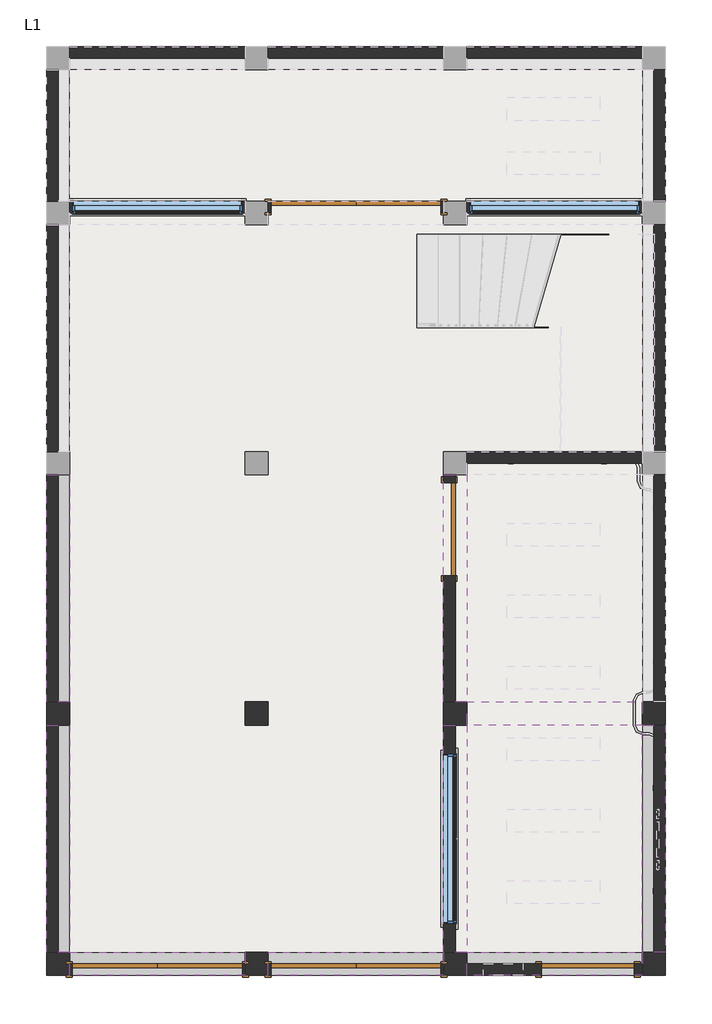
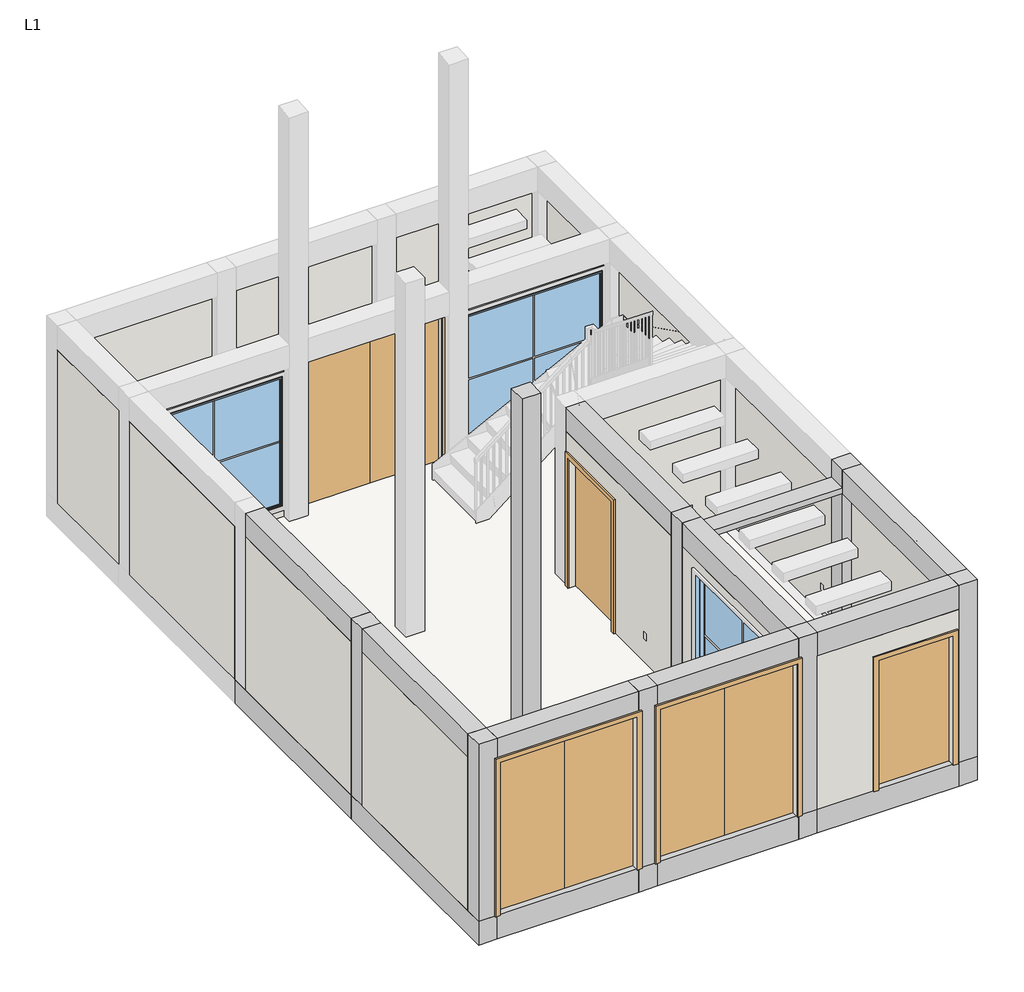
# One storey, part 1 of 3: 22 beams, 20 walls, 8 columns, 5 doors, 3 windows, 1 slab.
"""IFC4 building model written with IfcOpenShell, lengths in millimetres."""

import ifcopenshell
import ifcopenshell.guid

model = None  # the IFC model being written
_history = None  # IfcOwnerHistory: only IFC2X3 demands one
_inside = {}  # id of a spatial element -> (the spatial element, [elements in it])
_under = {}  # id of a project, library or spatial element -> (it, [spatial elements below it])
_declared = {}  # id of a project -> (the project, [libraries it declares])
_typed = {}  # id of a type object -> (the type object, [elements of that type])
_made_of = {}  # id of a material, layer set ... -> (it, [elements and type objects made of it])


def new_model(schema):
    """Start an empty IFC model of exactly this schema.

    Asked for "IFC4X3", IfcOpenShell would pick the latest addendum, in which some entities
    have other attributes; the version numbers below select the first issue.
    IFC2X3 requires an IfcOwnerHistory on every rooted entity: one is made here for all.
    """
    global model, _history
    if schema == "IFC4X3":
        model = ifcopenshell.file(schema_version=(4, 3, 0, 0))
    else:
        model = ifcopenshell.file(schema=schema)
    _inside.clear()
    _under.clear()
    _declared.clear()
    _typed.clear()
    _made_of.clear()
    _history = None
    if model.schema == "IFC2X3":
        org = make("IfcOrganization", Name="unknown")
        user = make(
            "IfcPersonAndOrganization",
            ThePerson=make("IfcPerson", FamilyName="unknown"),
            TheOrganization=org,
        )
        app = make(
            "IfcApplication",
            ApplicationDeveloper=org,
            Version="unknown",
            ApplicationFullName="unknown",
            ApplicationIdentifier="unknown",
        )
        _history = make(
            "IfcOwnerHistory",
            OwningUser=user,
            OwningApplication=app,
            ChangeAction="ADDED",
            CreationDate=0,
        )
    return model


def make(cls, **values):
    """One entity of the class cls with the attributes given. An attribute that is None is left unset."""
    return model.create_entity(
        cls, **{name: value for name, value in values.items() if value is not None}
    )


def rooted(cls, **values):
    """An entity with a GlobalId (a new one), such as an element, a storey or a relation."""
    return make(cls, GlobalId=ifcopenshell.guid.new(), OwnerHistory=_history, **values)


def si_unit(unit_type, name, prefix=None):
    """IfcSIUnit, for example si_unit("LENGTHUNIT", "METRE", prefix="MILLI")."""
    return make("IfcSIUnit", UnitType=unit_type, Prefix=prefix, Name=name)


def assignment(units):
    """IfcUnitAssignment: the units of a project."""
    return None if units is None else make("IfcUnitAssignment", Units=units)


def point(xyz):
    """IfcCartesianPoint."""
    return None if xyz is None else make("IfcCartesianPoint", Coordinates=xyz)


def direction(xyz):
    """IfcDirection."""
    return None if xyz is None else make("IfcDirection", DirectionRatios=xyz)


def frame(location, z_axis=None, x_axis=None):
    """IfcAxis2Placement3D, a coordinate frame: its origin and axes. An axis left out is left unset."""
    return make(
        "IfcAxis2Placement3D",
        Location=point(location),
        Axis=direction(z_axis),
        RefDirection=direction(x_axis),
    )


def origin():
    """The frame at (0, 0, 0) with its axes left unset."""
    return frame((0.0, 0.0, 0.0))


def origin_with_axes():
    """The frame at (0, 0, 0) with the z axis (0, 0, 1) and the x axis (1, 0, 0) written out."""
    return frame((0.0, 0.0, 0.0), z_axis=(0.0, 0.0, 1.0), x_axis=(1.0, 0.0, 0.0))


def place(relative_to, where):
    """IfcLocalPlacement: puts the frame where relative to a parent placement (None: the world)."""
    return make(
        "IfcLocalPlacement", PlacementRelTo=relative_to, RelativePlacement=where
    )


def context(
    kind, dimensions, precision=None, world=None, true_north=None, identifier=None
):
    """IfcGeometricRepresentationContext, for example the 3D "Model" context."""
    return make(
        "IfcGeometricRepresentationContext",
        ContextIdentifier=identifier,
        ContextType=kind,
        CoordinateSpaceDimension=dimensions,
        Precision=precision,
        WorldCoordinateSystem=world,
        TrueNorth=true_north,
    )


def project(units=None, contexts=None):
    """IfcProject with its units and contexts."""
    return rooted(
        "IfcProject",
        Name="project",
        RepresentationContexts=contexts,
        UnitsInContext=assignment(units),
    )


def spatial(cls, under=None, at=None, **own):
    """A site, building, storey or space (cls), placed at a placement, below another one or the project."""
    s = rooted(cls, ObjectPlacement=at, **own)
    if under is not None:
        _under.setdefault(under.id(), (under, []))[1].append(s)
    return s


def polyline(points):
    """IfcPolyline through the points."""
    return make("IfcPolyline", Points=[point(p) for p in points])


def outline(outer, holes=None, kind="AREA"):
    """IfcArbitraryClosedProfileDef: a profile drawn as a closed curve; with holes, ...WithVoids."""
    if holes is None:
        return make("IfcArbitraryClosedProfileDef", ProfileType=kind, OuterCurve=outer)
    return make(
        "IfcArbitraryProfileDefWithVoids",
        ProfileType=kind,
        OuterCurve=outer,
        InnerCurves=holes,
    )


def extrude(swept, where, along, depth):
    """IfcExtrudedAreaSolid: the profile swept, set in the frame where, extruded along a direction by depth."""
    return make(
        "IfcExtrudedAreaSolid",
        SweptArea=swept,
        Position=where,
        ExtrudedDirection=direction(along),
        Depth=depth,
    )


def faces_of(points, faces, orient=None, outer=None):
    """IfcFace entities. A face is a list of loops; a loop is a list of indices into points, from 0.

    orient and outer hold one flag for each loop. By default every Orientation is true, the
    first loop of a face is its IfcFaceOuterBound and the others are IfcFaceBound.
    """
    made = []
    for i, loops in enumerate(faces):
        bounds = []
        for j, loop in enumerate(loops):
            is_outer = j == 0 if outer is None else outer[i][j]
            bounds.append(
                make(
                    "IfcFaceOuterBound" if is_outer else "IfcFaceBound",
                    Bound=make("IfcPolyLoop", Polygon=[points[k] for k in loop]),
                    Orientation=True if orient is None else orient[i][j],
                )
            )
        made.append(make("IfcFace", Bounds=bounds))
    return made


def faceted_brep(points, faces, orient=None, outer=None, voids=None):
    """IfcFacetedBrep: a solid bounded by flat faces; with voids (closed shells), ...WithVoids."""
    shared = [point(p) for p in points]
    hull = make("IfcClosedShell", CfsFaces=faces_of(shared, faces, orient, outer))
    if voids is None:
        return make("IfcFacetedBrep", Outer=hull)
    return make(
        "IfcFacetedBrepWithVoids",
        Outer=hull,
        Voids=[
            make(cls, CfsFaces=faces_of(shared, fs, o, b)) for cls, fs, o, b in voids
        ],
    )


def shape(context_of_items, identifier, shape_type, items):
    """IfcShapeRepresentation: the items that make up one representation, for example the "Body"."""
    return make(
        "IfcShapeRepresentation",
        ContextOfItems=context_of_items,
        RepresentationIdentifier=identifier,
        RepresentationType=shape_type,
        Items=items,
    )


def source(mapping_origin, context_of_items, identifier, shape_type, items):
    """IfcRepresentationMap: a shape defined once, which mapped items show again and again."""
    return make(
        "IfcRepresentationMap",
        MappingOrigin=mapping_origin,
        MappedRepresentation=shape(context_of_items, identifier, shape_type, items),
    )


def transform(
    local_origin,
    x_axis=None,
    y_axis=None,
    z_axis=None,
    scale=None,
    scale2=None,
    scale3=None,
    uniform=True,
):
    """IfcCartesianTransformationOperator3D, or its non-uniform kind. x_axis, y_axis, z_axis: its Axis1, 2, 3."""
    if uniform:
        return make(
            "IfcCartesianTransformationOperator3D",
            Axis1=direction(x_axis),
            Axis2=direction(y_axis),
            LocalOrigin=point(local_origin),
            Scale=scale,
            Axis3=direction(z_axis),
        )
    return make(
        "IfcCartesianTransformationOperator3DnonUniform",
        Axis1=direction(x_axis),
        Axis2=direction(y_axis),
        LocalOrigin=point(local_origin),
        Scale=scale,
        Axis3=direction(z_axis),
        Scale2=scale2,
        Scale3=scale3,
    )


def mapped(mapping_source, mapping_target):
    """IfcMappedItem: shows the shape of a source again, moved by a transform."""
    return make(
        "IfcMappedItem", MappingSource=mapping_source, MappingTarget=mapping_target
    )


def made_of(thing, what):
    """Note that an element or type object is made of a material, layer set ...; save() writes the relation."""
    if what is not None:
        _made_of.setdefault(what.id(), (what, []))[1].append(thing)
    return thing


def element(
    cls,
    number,
    at=None,
    inside=None,
    cuts=None,
    type_object=None,
    material=None,
    context=None,
    identifier="Body",
    shape_type=None,
    held_by="IfcProductDefinitionShape",
    body=None,
    shapes=None,
    **own,
):
    """One element of the class cls, such as IfcWall. Its Tag is "e" and its number.

    at: its placement. inside: the storey or other place that contains it. cuts: it is an
    opening in that element (IfcRelVoidsElement). A single representation is given by context,
    identifier, shape_type and body (its items); several are given by shapes. held_by: the class
    of the entity that holds the representations. save() writes the other relations.
    """
    e = rooted(cls, Tag="e%d" % number, ObjectPlacement=at, **own)
    if body is not None:
        shapes = [shape(context, identifier, shape_type, body)]
    if shapes is not None:
        e.Representation = make(held_by, Representations=shapes)
    if inside is not None:
        _inside.setdefault(inside.id(), (inside, []))[1].append(e)
    if cuts is not None:
        rooted(
            "IfcRelVoidsElement", RelatingBuildingElement=cuts, RelatedOpeningElement=e
        )
    if type_object is not None:
        _typed.setdefault(type_object.id(), (type_object, []))[1].append(e)
    return made_of(e, material)


def aggregate(whole, parts):
    """IfcRelAggregates: a whole, such as a stair, and the parts it consists of."""
    return rooted("IfcRelAggregates", RelatingObject=whole, RelatedObjects=parts)


def save(model, path):
    """Write the relations noted so far, then the file.

    IfcRelAggregates (storeys below a building ...), IfcRelContainedInSpatialStructure (elements
    in a storey), IfcRelDefinesByType, IfcRelAssociatesMaterial and IfcRelDeclares: one each for
    every whole, place, type object, material and project.
    """
    for whole, parts in _under.values():
        aggregate(whole, parts)
    for where, things in _inside.values():
        rooted(
            "IfcRelContainedInSpatialStructure",
            RelatedElements=things,
            RelatingStructure=where,
        )
    for kind, things in _typed.values():
        rooted("IfcRelDefinesByType", RelatedObjects=things, RelatingType=kind)
    for what, things in _made_of.values():
        rooted("IfcRelAssociatesMaterial", RelatedObjects=things, RelatingMaterial=what)
    for by, libraries in _declared.values():
        rooted("IfcRelDeclares", RelatingContext=by, RelatedDefinitions=libraries)
    model.write(path)


def door_double_flush_panel_2_2_x_2_6_m_98fec84c(model_context):
    return source(origin(), model_context, "Body", "SweptSolid", [
        extrude(outline(polyline([(2600.0, -1100.0), (2600.0, 1100.0), (0.0, 1100.0), (0.0, 1176.2), (2676.2, 1176.2), (2676.2, -1176.2), (0.0, -1176.2), (0.0, -1100.0), (2600.0, -1100.0)])), frame((0.0, 75.0, 0.0), z_axis=(0.0, 1.0, 0.0), x_axis=(0.0, 0.0, 1.0)), (0.0, 0.0, 1.0), 25.4),
        extrude(outline(polyline([(2600.0, -1100.0), (2600.0, 1100.0), (0.0, 1100.0), (0.0, 1176.2), (2676.2, 1176.2), (2676.2, -1176.2), (0.0, -1176.2), (0.0, -1100.0), (2600.0, -1100.0)])), frame((0.0, -100.4, 0.0), z_axis=(0.0, 1.0, 0.0), x_axis=(0.0, 0.0, 1.0)), (0.0, 0.0, 1.0), 25.4),
        extrude(outline(polyline([(-1100.0, 75.0), (0.0, 75.0), (0.0, 24.2), (-1100.0, 24.2), (-1100.0, 75.0)])), origin_with_axes(), (0.0, 0.0, 1.0), 2600.0),
        extrude(outline(polyline([(0.0, 75.0), (1100.0, 75.0), (1100.0, 24.2), (0.0, 24.2), (0.0, 75.0)])), origin_with_axes(), (0.0, 0.0, 1.0), 2600.0),
    ])


def door_single_panel_1_2_x_2_2_m_37493633(model_context):
    return source(origin(), model_context, "Body", "SweptSolid", [
        extrude(outline(polyline([(600.0, 24.2), (-600.0, 24.2), (-600.0, 75.0), (600.0, 75.0), (600.0, 24.2)])), origin_with_axes(), (0.0, 0.0, 1.0), 2200.0),
        extrude(outline(polyline([(2276.2, 676.2), (2276.2, -676.2), (0.0, -676.2), (0.0, -600.0), (2200.0, -600.0), (2200.0, 600.0), (0.0, 600.0), (0.0, 676.2), (2276.2, 676.2)])), frame((0.0, -100.4, 0.0), z_axis=(0.0, 1.0, 0.0), x_axis=(0.0, 0.0, 1.0)), (0.0, 0.0, 1.0), 25.4),
        extrude(outline(polyline([(2276.2, -676.2), (0.0, -676.2), (0.0, -600.0), (2200.0, -600.0), (2200.0, 600.0), (0.0, 600.0), (0.0, 676.2), (2276.2, 676.2), (2276.2, -676.2)])), frame((0.0, 75.0, 0.0), z_axis=(0.0, 1.0, 0.0), x_axis=(0.0, 0.0, 1.0)), (0.0, 0.0, 1.0), 25.4),
    ])


def door_single_panel_1_2_x_2_2_m_3fbad9d7(model_context):
    return source(origin(), model_context, "Body", "SweptSolid", [
        extrude(outline(polyline([(600.0, -24.2), (600.0, -75.0), (-600.0, -75.0), (-600.0, -24.2), (600.0, -24.2)])), origin_with_axes(), (0.0, 0.0, 1.0), 2200.0),
        extrude(outline(polyline([(2276.2, 676.2), (2276.2, -676.2), (0.0, -676.2), (0.0, -600.0), (2200.0, -600.0), (2200.0, 600.0), (0.0, 600.0), (0.0, 676.2), (2276.2, 676.2)])), frame((0.0, 75.0, 0.0), z_axis=(0.0, 1.0, 0.0), x_axis=(0.0, 0.0, 1.0)), (0.0, 0.0, 1.0), 25.4),
        extrude(outline(polyline([(2276.2, -676.2), (0.0, -676.2), (0.0, -600.0), (2200.0, -600.0), (2200.0, 600.0), (0.0, 600.0), (0.0, 676.2), (2276.2, 676.2), (2276.2, -676.2)])), frame((0.0, -100.4, 0.0), z_axis=(0.0, 1.0, 0.0), x_axis=(0.0, 0.0, 1.0)), (0.0, 0.0, 1.0), 25.4),
    ])


def window_fixed_2_2_x_2_2_m_8ae7ec15(model_context):
    return source(origin(), model_context, "Body", "SolidModel", [
        faceted_brep([(1100.0, -20.25, 3114.4), (1100.0, 94.05, 3114.4), (-1100.0, 94.05, 3114.4), (-1100.0, -20.25, 3114.4), (-1100.0, 94.05, 914.4), (-1100.0, -20.25, 914.4), (1100.0, 94.05, 914.4), (1100.0, -20.25, 914.4), (1068.25, -20.25, 3082.65), (1068.25, -20.25, 946.15), (-1068.25, -20.25, 946.15), (-1068.25, -20.25, 3082.65), (-1087.3, 94.05, 3101.7), (-1087.3, 94.05, 927.1), (1087.3, 94.05, 927.1), (1087.3, 94.05, 3101.7), (1068.25, 43.25, 3082.65), (-1068.25, 43.25, 3082.65), (1087.3, 43.25, 3101.7), (-1087.3, 43.25, 3101.7), (-1068.25, 43.25, 946.15), (-1087.3, 43.25, 927.1), (1068.25, 43.25, 946.15), (1087.3, 43.25, 927.1)], [[[0, 1, 2, 3]], [[3, 2, 4, 5]], [[5, 4, 6, 7]], [[3, 5, 7, 0], [8, 9, 10, 11]], [[7, 6, 1, 0]], [[1, 6, 4, 2], [12, 13, 14, 15]], [[16, 8, 11, 17]], [[15, 18, 19, 12]], [[17, 11, 10, 20]], [[12, 19, 21, 13]], [[20, 10, 9, 22]], [[13, 21, 23, 14]], [[22, 9, 8, 16]], [[18, 23, 21, 19], [17, 20, 22, 16]], [[14, 23, 18, 15]]]),
        extrude(outline(polyline([(3114.4, -1100.0), (914.4, -1100.0), (914.4, 1100.0), (3114.4, 1100.0), (3114.4, -1100.0)]), holes=[polyline([(3101.7, 1087.3), (927.1, 1087.3), (927.1, -1087.3), (3101.7, -1087.3), (3101.7, 1087.3)])]), frame((0.0, -75.0, 0.0), z_axis=(0.0, 1.0, 0.0), x_axis=(0.0, 0.0, 1.0)), (0.0, 0.0, 1.0), 54.75),
        extrude(outline(polyline([(927.1, 1087.3), (3101.7, 1087.3), (3101.7, -1087.3), (927.1, -1087.3), (927.1, 1087.3)]), holes=[polyline([(952.5, -1061.9), (3076.3, -1061.9), (3076.3, 1061.9), (952.5, 1061.9), (952.5, -1061.9)])]), frame((0.0, 43.25, 0.0), z_axis=(0.0, 1.0, 0.0), x_axis=(0.0, 0.0, 1.0)), (0.0, 0.0, 1.0), 44.45),
        extrude(outline(polyline([(1061.9, 75.0), (1061.9, 68.65), (-1061.9, 68.65), (-1061.9, 75.0), (1061.9, 75.0)])), frame((0.0, 0.0, 952.5), z_axis=(0.0, 0.0, 1.0), x_axis=(1.0, 0.0, 0.0)), (0.0, 0.0, 1.0), 2123.8),
        extrude(outline(polyline([(-1061.9, 55.95), (-1061.9, 62.3), (1061.9, 62.3), (1061.9, 55.95), (-1061.9, 55.95)])), frame((0.0, 0.0, 952.5), z_axis=(0.0, 0.0, 1.0), x_axis=(1.0, 0.0, 0.0)), (0.0, 0.0, 1.0), 2123.8),
    ])


model = new_model("IFC4")

# Units and contexts
model_context = context("Model", 3, world=origin())
ifc_project = project(units=[si_unit("LENGTHUNIT", "METRE", prefix="MILLI")], contexts=[model_context])

# Site, building, storey
site = spatial("IfcSite", under=ifc_project)
building = spatial("IfcBuilding", under=site)
storey = spatial("IfcBuildingStorey", under=building, Name="L1", Elevation=0.0)

# Beams
placement = place(None, origin())
element("IfcBeam", 1, ObjectType="Concrete-Rectangular Beam : 30 x 40 cm", at=placement, inside=storey, context=model_context, shape_type="Brep", body=[
    faceted_brep([(-4000.0, -5500.0, 0.0), (-3700.0, -5500.0, 0.0), (-3700.0, -5200.0, 0.0), (-3700.0, -2266.6666663, 0.0), (-3700.0, -1966.6666663, 0.0), (-4000.0, -1966.6666663, 0.0), (-4000.0, -2266.6666663, 0.0), (-4000.0, -5200.0, 0.0), (-3700.0, -5500.0, -400.0), (-3700.0, -5200.0, -400.0), (-3700.0, -2266.6666663, -400.0), (-3700.0, -1966.6666663, -400.0), (-3700.0, -1966.6666663, -300.0), (-4000.0, -5500.0, -400.0), (-4000.0, -1966.6666663, -400.0)], [[[0, 1, 2, 3, 4, 5, 6, 7]], [[1, 8, 9, 10, 11, 12, 4, 3, 2]], [[8, 13, 14, 11, 10, 9]], [[13, 0, 7, 6, 5, 14]], [[1, 0, 13, 8]], [[5, 4, 12, 11, 14]]]),
])
element("IfcBeam", 2, ObjectType="Concrete-Rectangular Beam : 30 x 40 cm", at=placement, inside=storey, context=model_context, shape_type="Brep", body=[
    faceted_brep([(-3700.0, 1266.666667, 0.0), (-4000.0, 1266.666667, 0.0), (-4000.0, 966.666667, 0.0), (-4000.0, -1966.6666663, 0.0), (-3700.0, -1966.6666663, 0.0), (-3700.0, 966.666667, 0.0), (-3700.0, 1266.666667, -400.0), (-3700.0, 1266.666667, -300.0), (-3700.0, -1966.6666663, -400.0), (-3700.0, 966.666667, -400.0), (-4000.0, 1266.666667, -400.0), (-4000.0, -1966.6666663, -400.0)], [[[0, 1, 2, 3, 4, 5]], [[6, 7, 0, 5, 4, 8, 9]], [[10, 6, 9, 8, 11]], [[1, 10, 11, 3, 2]], [[1, 0, 7, 6, 10]], [[4, 3, 11, 8]]]),
])
element("IfcBeam", 3, ObjectType="Concrete-Rectangular Beam : 30 x 40 cm", at=placement, inside=storey, context=model_context, shape_type="Brep", body=[
    faceted_brep([(-1433.3333333, -5500.0, 0.0), (-1133.3333333, -5500.0, 0.0), (-1133.3333333, -5200.0, 0.0), (-1433.3333333, -5200.0, 0.0), (-1133.3333333, -5500.0, -400.0), (-1133.3333333, -5200.0, -400.0), (-1133.3333333, -2266.6666663, -400.0), (-1133.3333333, -1966.6666663, -400.0), (-1133.3333333, -1966.6666663, -300.0), (-1133.3333333, -2266.6666663, -300.0), (-1133.3333333, -5200.0, -300.0), (-1433.3333333, -5500.0, -400.0), (-1433.3333333, -5200.0, -400.0), (-1433.3333333, -2266.6666663, -400.0), (-1433.3333333, -1966.6666663, -400.0), (-1433.3333333, -5200.0, -300.0), (-1433.3333333, -2266.6666663, -300.0), (-1433.3333333, -1966.6666663, -300.0)], [[[0, 1, 2, 3]], [[1, 4, 5, 6, 7, 8, 9, 10, 2]], [[4, 11, 12, 13, 14, 7, 6, 5]], [[11, 0, 3, 15, 16, 17, 14, 13, 12]], [[1, 0, 11, 4]], [[7, 14, 17, 8]], [[15, 10, 9, 8, 17, 16]], [[10, 15, 3, 2]]]),
])
element("IfcBeam", 4, ObjectType="Concrete-Rectangular Beam : 30 x 40 cm", at=placement, inside=storey, context=model_context, shape_type="Brep", body=[
    faceted_brep([(-1133.3333333, -1966.6666663, -400.0), (-1133.3333333, 966.666667, -400.0), (-1133.3333333, 1266.666667, -400.0), (-1133.3333333, 1266.666667, -300.0), (-1133.3333333, 966.666667, -300.0), (-1133.3333333, -1966.6666663, -300.0), (-1433.3333333, 1266.666667, -400.0), (-1433.3333333, -1966.6666663, -400.0), (-1433.3333333, 966.666667, -400.0), (-1433.3333333, -1966.6666663, -300.0), (-1433.3333333, 966.666667, -300.0), (-1433.3333333, 1266.666667, -300.0)], [[[0, 1, 2, 3, 4, 5]], [[6, 2, 1, 0, 7, 8]], [[6, 8, 7, 9, 10, 11]], [[2, 6, 11, 3]], [[7, 0, 5, 9]], [[5, 4, 3, 11, 10, 9]]]),
])
element("IfcBeam", 5, ObjectType="Concrete-Rectangular Beam : 30 x 40 cm", at=placement, inside=storey, context=model_context, shape_type="Brep", body=[
    faceted_brep([(1133.33334, -5500.0, 0.0), (1433.33334, -5500.0, 0.0), (1433.33334, -5200.0, 0.0), (1133.33334, -5200.0, 0.0), (1433.33334, -5500.0, -400.0), (1433.33334, -5200.0, -400.0), (1433.33334, -2266.6666663, -400.0), (1433.33334, -1966.6666663, -400.0), (1433.33334, -1966.6666663, -300.0), (1433.33334, -2266.6666663, -300.0), (1433.33334, -5200.0, -300.0), (1133.33334, -5500.0, -400.0), (1133.33334, -5200.0, -400.0), (1133.33334, -2266.6666663, -400.0), (1133.33334, -1966.6666663, -400.0), (1133.33334, -5200.0, -300.0), (1133.33334, -2266.6666663, -300.0), (1133.33334, -1966.6666663, -300.0)], [[[0, 1, 2, 3]], [[1, 4, 5, 6, 7, 8, 9, 10, 2]], [[4, 11, 12, 13, 14, 7, 6, 5]], [[11, 0, 3, 15, 16, 17, 14, 13, 12]], [[1, 0, 11, 4]], [[7, 14, 17, 8]], [[15, 10, 9, 8, 17, 16]], [[10, 15, 3, 2]]]),
])
element("IfcBeam", 6, ObjectType="Concrete-Rectangular Beam : 30 x 40 cm", at=placement, inside=storey, context=model_context, shape_type="Brep", body=[
    faceted_brep([(1433.33334, -1966.6666663, -400.0), (1433.33334, 966.666667, -400.0), (1433.33334, 1266.666667, -400.0), (1433.33334, 1266.666667, -300.0), (1433.33334, 966.666667, -300.0), (1433.33334, -1966.6666663, -300.0), (1133.33334, 1266.666667, -400.0), (1133.33334, -1966.6666663, -400.0), (1133.33334, 966.666667, -400.0), (1133.33334, -1966.6666663, -300.0), (1133.33334, 966.666667, -300.0), (1133.33334, 1266.666667, -300.0)], [[[0, 1, 2, 3, 4, 5]], [[6, 2, 1, 0, 7, 8]], [[6, 8, 7, 9, 10, 11]], [[2, 6, 11, 3]], [[7, 0, 5, 9]], [[5, 4, 3, 11, 10, 9]]]),
])
element("IfcBeam", 7, ObjectType="Concrete-Rectangular Beam : 30 x 40 cm", at=placement, inside=storey, context=model_context, shape_type="Brep", body=[
    faceted_brep([(3700.0, -5500.0, 0.0), (4000.0, -5500.0, 0.0), (4000.0, -1966.6666663, 0.0), (3700.0, -1966.6666663, 0.0), (3700.0, -5200.0, 0.0), (4000.0, -5500.0, -400.0), (4000.0, -1966.6666663, -400.0), (3700.0, -5500.0, -400.0), (3700.0, -5200.0, -400.0), (3700.0, -2266.6666663, -400.0), (3700.0, -1966.6666663, -400.0), (3700.0, -1966.6666663, -300.0)], [[[0, 1, 2, 3, 4]], [[1, 5, 6, 2]], [[5, 7, 8, 9, 10, 6]], [[7, 0, 4, 3, 11, 10, 9, 8]], [[1, 0, 7, 5]], [[3, 2, 6, 10, 11]]]),
])
element("IfcBeam", 8, ObjectType="Concrete-Rectangular Beam : 30 x 40 cm", at=placement, inside=storey, context=model_context, shape_type="SweptSolid", body=[
    extrude(outline(polyline([(1433.33334, -2266.6666663), (1433.33334, -1966.6666663), (3700.0, -1966.6666663), (3700.0, -2266.6666663), (1433.33334, -2266.6666663)])), frame((0.0, 0.0, -400.0), z_axis=(0.0, 0.0, 1.0), x_axis=(1.0, 0.0, 0.0)), (0.0, 0.0, 1.0), 100.0),
])
element("IfcBeam", 9, ObjectType="Concrete-Rectangular Beam : 30 x 40 cm", at=placement, inside=storey, context=model_context, shape_type="SweptSolid", body=[
    extrude(outline(polyline([(-1133.3333333, -2266.6666663), (-1133.3333333, -1966.6666663), (1133.33334, -1966.6666663), (1133.33334, -2266.6666663), (-1133.3333333, -2266.6666663)])), frame((0.0, 0.0, -400.0), z_axis=(0.0, 0.0, 1.0), x_axis=(1.0, 0.0, 0.0)), (0.0, 0.0, 1.0), 100.0),
])
element("IfcBeam", 10, ObjectType="Concrete-Rectangular Beam : 30 x 40 cm", at=placement, inside=storey, context=model_context, shape_type="SweptSolid", body=[
    extrude(outline(polyline([(-3700.0, -2266.6666663), (-3700.0, -1966.6666663), (-1433.3333333, -1966.6666663), (-1433.3333333, -2266.6666663), (-3700.0, -2266.6666663)])), frame((0.0, 0.0, -400.0), z_axis=(0.0, 0.0, 1.0), x_axis=(1.0, 0.0, 0.0)), (0.0, 0.0, 1.0), 100.0),
])
element("IfcBeam", 11, ObjectType="Concrete-Rectangular Beam : 30 x 40 cm", at=placement, inside=storey, context=model_context, shape_type="Brep", body=[
    faceted_brep([(1433.33334, -5200.0, 0.0), (1433.33334, -5500.0, 0.0), (3700.0, -5500.0, 0.0), (3700.0, -5200.0, 0.0), (1433.33334, -5200.0, -400.0), (1433.33334, -5200.0, -300.0), (3700.0, -5200.0, -300.0), (3700.0, -5200.0, -400.0), (1433.33334, -5500.0, -400.0), (3700.0, -5500.0, -400.0)], [[[0, 1, 2, 3]], [[4, 5, 0, 3, 6, 7]], [[8, 4, 7, 9]], [[1, 8, 9, 2]], [[1, 0, 5, 4, 8]], [[3, 2, 9, 7, 6]]]),
])
element("IfcBeam", 12, ObjectType="Concrete-Rectangular Beam : 30 x 40 cm", at=placement, inside=storey, context=model_context, shape_type="Brep", body=[
    faceted_brep([(-1133.3333333, -5200.0, 0.0), (-1133.3333333, -5500.0, 0.0), (1133.33334, -5500.0, 0.0), (1133.33334, -5200.0, 0.0), (-1133.3333333, -5200.0, -400.0), (-1133.3333333, -5200.0, -300.0), (1133.33334, -5200.0, -300.0), (1133.33334, -5200.0, -400.0), (-1133.3333333, -5500.0, -400.0), (1133.33334, -5500.0, -400.0)], [[[0, 1, 2, 3]], [[4, 5, 0, 3, 6, 7]], [[8, 4, 7, 9]], [[1, 8, 9, 2]], [[1, 0, 5, 4, 8]], [[3, 2, 9, 7, 6]]]),
])
element("IfcBeam", 13, ObjectType="Concrete-Rectangular Beam : 30 x 40 cm", at=placement, inside=storey, context=model_context, shape_type="Brep", body=[
    faceted_brep([(-3700.0, -5200.0, 0.0), (-3700.0, -5500.0, 0.0), (-1433.3333333, -5500.0, 0.0), (-1433.3333333, -5200.0, 0.0), (-3700.0, -5200.0, -400.0), (-3700.0, -5200.0, -300.0), (-1433.3333333, -5200.0, -300.0), (-1433.3333333, -5200.0, -400.0), (-3700.0, -5500.0, -400.0), (-1433.3333333, -5500.0, -400.0)], [[[0, 1, 2, 3]], [[4, 5, 0, 3, 6, 7]], [[8, 4, 7, 9]], [[1, 8, 9, 2]], [[1, 0, 5, 4, 8]], [[3, 2, 9, 7, 6]]]),
])
element("IfcBeam", 14, ObjectType="Concrete-Rectangular Beam : 30 x 40 cm", at=placement, inside=storey, context=model_context, shape_type="SweptSolid", body=[
    extrude(outline(polyline([(-4000.0, -2266.6666663), (-3700.0, -2266.6666663), (-3700.0, -5200.0), (-4000.0, -5200.0), (-4000.0, -2266.6666663)])), frame((0.0, 0.0, 2600.0), z_axis=(0.0, 0.0, 1.0), x_axis=(1.0, 0.0, 0.0)), (0.0, 0.0, 1.0), 400.0),
])
element("IfcBeam", 15, ObjectType="Concrete-Rectangular Beam : 30 x 40 cm", at=placement, inside=storey, context=model_context, shape_type="SweptSolid", body=[
    extrude(outline(polyline([(-4000.0, 966.666667), (-3700.0, 966.666667), (-3700.0, -1966.6666663), (-4000.0, -1966.6666663), (-4000.0, 966.666667)])), frame((0.0, 0.0, 2600.0), z_axis=(0.0, 0.0, 1.0), x_axis=(1.0, 0.0, 0.0)), (0.0, 0.0, 1.0), 400.0),
])
element("IfcBeam", 16, ObjectType="Concrete-Rectangular Beam : 30 x 40 cm", at=placement, inside=storey, context=model_context, shape_type="Brep", body=[
    faceted_brep([(1433.33334, -2266.6666663, 3000.0), (1133.33334, -2266.6666663, 3000.0), (1133.33334, -5200.0, 3000.0), (1433.33334, -5200.0, 3000.0), (1433.33334, -2266.6666663, 2600.0), (1433.33334, -5200.0, 2700.0), (1433.33334, -5200.0, 2600.0), (1133.33334, -2266.6666663, 2600.0), (1133.33334, -5200.0, 2600.0)], [[[0, 1, 2, 3]], [[4, 0, 3, 5, 6]], [[7, 4, 6, 8]], [[1, 7, 8, 2]], [[1, 0, 4, 7]], [[3, 2, 8, 6, 5]]]),
])
element("IfcBeam", 17, ObjectType="Concrete-Rectangular Beam : 30 x 40 cm", at=placement, inside=storey, context=model_context, shape_type="Brep", body=[
    faceted_brep([(1433.33334, 966.666667, 3000.0), (1133.33334, 966.666667, 3000.0), (1133.33334, -1966.6666663, 3000.0), (1433.33334, -1966.6666663, 3000.0), (1433.33334, 966.666667, 2600.0), (1433.33334, 966.666667, 2700.0), (1433.33334, -1966.6666663, 2600.0), (1133.33334, 966.666667, 2600.0), (1133.33334, -1966.6666663, 2600.0)], [[[0, 1, 2, 3]], [[4, 5, 0, 3, 6]], [[7, 4, 6, 8]], [[1, 7, 8, 2]], [[1, 0, 5, 4, 7]], [[2, 8, 6, 3]]]),
])
element("IfcBeam", 18, ObjectType="Concrete-Rectangular Beam : 30 x 40 cm", at=placement, inside=storey, context=model_context, shape_type="Brep", body=[
    faceted_brep([(4000.0, -2266.6666663, 3000.0), (3700.0, -2266.6666663, 3000.0), (3700.0, -5200.0, 3000.0), (4000.0, -5200.0, 3000.0), (4000.0, -2266.6666663, 2600.0), (4000.0, -5200.0, 2600.0), (3700.0, -2266.6666663, 2600.0), (3700.0, -5200.0, 2600.0), (3700.0, -5200.0, 2700.0)], [[[0, 1, 2, 3]], [[4, 0, 3, 5]], [[6, 4, 5, 7]], [[1, 6, 7, 8, 2]], [[1, 0, 4, 6]], [[3, 2, 8, 7, 5]]]),
])
element("IfcBeam", 19, ObjectType="Concrete-Rectangular Beam : 30 x 40 cm", at=placement, inside=storey, context=model_context, shape_type="SweptSolid", body=[
    extrude(outline(polyline([(1433.33334, -2266.6666663), (1433.33334, -1966.6666663), (3699.9988976, -1966.6666663), (3699.9988976, -2266.6666663), (1433.33334, -2266.6666663)])), frame((0.0, 0.0, 2600.0), z_axis=(0.0, 0.0, 1.0), x_axis=(1.0, 0.0, 0.0)), (0.0, 0.0, 1.0), 100.0),
])
element("IfcBeam", 20, ObjectType="Concrete-Rectangular Beam : 30 x 40 cm", at=placement, inside=storey, context=model_context, shape_type="Brep", body=[
    faceted_brep([(1433.33334, -5200.0, 3000.0), (1433.33334, -5500.0, 3000.0), (3699.9988976, -5500.0, 3000.0), (3699.9988976, -5200.0, 3000.0), (1433.33334, -5200.0, 2600.0), (1433.33334, -5200.0, 2700.0), (3699.9988976, -5200.0, 2600.0), (1433.33334, -5500.0, 2600.0), (3699.9988976, -5500.0, 2600.0)], [[[0, 1, 2, 3]], [[4, 5, 0, 3, 6]], [[7, 4, 6, 8]], [[1, 7, 8, 2]], [[1, 0, 5, 4, 7]], [[3, 2, 8, 6]]]),
])
element("IfcBeam", 21, ObjectType="Concrete-Rectangular Beam : 30 x 40 cm", at=placement, inside=storey, context=model_context, shape_type="SweptSolid", body=[
    extrude(outline(polyline([(-1133.3333333, -5500.0), (-1133.3333333, -5200.0), (1133.33334, -5200.0), (1133.33334, -5500.0), (-1133.3333333, -5500.0)])), frame((0.0, 0.0, 2600.0), z_axis=(0.0, 0.0, 1.0), x_axis=(1.0, 0.0, 0.0)), (0.0, 0.0, 1.0), 400.0),
])
element("IfcBeam", 22, ObjectType="Concrete-Rectangular Beam : 30 x 40 cm", at=placement, inside=storey, context=model_context, shape_type="SweptSolid", body=[
    extrude(outline(polyline([(-3700.0, -5500.0), (-3700.0, -5200.0), (-1433.3333333, -5200.0), (-1433.3333333, -5500.0), (-3700.0, -5500.0)])), frame((0.0, 0.0, 2600.0), z_axis=(0.0, 0.0, 1.0), x_axis=(1.0, 0.0, 0.0)), (0.0, 0.0, 1.0), 400.0),
])

# Columns
element("IfcColumn", 23, ObjectType="Concrete-Square-Column : 30 x 30 cm", at=placement, inside=storey, context=model_context, shape_type="SweptSolid", body=[
    extrude(outline(polyline([(-4000.0, -2266.6666663), (-4000.0, -1966.6666663), (-3700.0, -1966.6666663), (-3700.0, -2266.6666663), (-4000.0, -2266.6666663)])), origin_with_axes(), (0.0, 0.0, 1.0), 3000.0),
])
element("IfcColumn", 24, ObjectType="Concrete-Square-Column : 30 x 30 cm", at=placement, inside=storey, context=model_context, shape_type="SweptSolid", body=[
    extrude(outline(polyline([(-1433.3333333, -2266.6666663), (-1433.3333333, -1966.6666663), (-1133.3333333, -1966.6666663), (-1133.3333333, -2266.6666663), (-1433.3333333, -2266.6666663)])), origin_with_axes(), (0.0, 0.0, 1.0), 6000.0),
])
element("IfcColumn", 25, ObjectType="Concrete-Square-Column : 30 x 30 cm", at=placement, inside=storey, context=model_context, shape_type="SweptSolid", body=[
    extrude(outline(polyline([(1133.33334, -2266.6666663), (1133.33334, -1966.6666663), (1433.33334, -1966.6666663), (1433.33334, -2266.6666663), (1133.33334, -2266.6666663)])), origin_with_axes(), (0.0, 0.0, 1.0), 3000.0),
])
element("IfcColumn", 26, ObjectType="Concrete-Square-Column : 30 x 30 cm", at=placement, inside=storey, context=model_context, shape_type="SweptSolid", body=[
    extrude(outline(polyline([(3699.9988976, -2266.6666663), (3699.9988976, -1966.6666663), (3999.9988976, -1966.6666663), (3999.9988976, -2266.6666663), (3699.9988976, -2266.6666663)])), origin_with_axes(), (0.0, 0.0, 1.0), 3000.0),
])
element("IfcColumn", 27, ObjectType="Concrete-Square-Column : 30 x 30 cm", at=placement, inside=storey, context=model_context, shape_type="SweptSolid", body=[
    extrude(outline(polyline([(-4000.0, -5500.0), (-4000.0, -5200.0), (-3700.0, -5200.0), (-3700.0, -5500.0), (-4000.0, -5500.0)])), origin_with_axes(), (0.0, 0.0, 1.0), 3000.0),
])
element("IfcColumn", 28, ObjectType="Concrete-Square-Column : 30 x 30 cm", at=placement, inside=storey, context=model_context, shape_type="SweptSolid", body=[
    extrude(outline(polyline([(-1433.3333333, -5500.0), (-1433.3333333, -5200.0), (-1133.3333333, -5200.0), (-1133.3333333, -5500.0), (-1433.3333333, -5500.0)])), origin_with_axes(), (0.0, 0.0, 1.0), 3000.0),
])
element("IfcColumn", 29, ObjectType="Concrete-Square-Column : 30 x 30 cm", at=placement, inside=storey, context=model_context, shape_type="SweptSolid", body=[
    extrude(outline(polyline([(1133.33334, -5500.0), (1133.33334, -5200.0), (1433.33334, -5200.0), (1433.33334, -5500.0), (1133.33334, -5500.0)])), origin_with_axes(), (0.0, 0.0, 1.0), 3000.0),
])
element("IfcColumn", 30, ObjectType="Concrete-Square-Column : 30 x 30 cm", at=placement, inside=storey, context=model_context, shape_type="SweptSolid", body=[
    extrude(outline(polyline([(3699.9988976, -5500.0), (3699.9988976, -5200.0), (3999.9988976, -5200.0), (3999.9988976, -5500.0), (3699.9988976, -5500.0)])), origin_with_axes(), (0.0, 0.0, 1.0), 3000.0),
])

# Doors
door_double_flush_panel_2_2_x_2_6_m_shape = door_double_flush_panel_2_2_x_2_6_m_98fec84c(model_context)
element("IfcDoor", 31, ObjectType="Door-Double-Flush_Panel : 2.2 x 2.6 m", at=placement, inside=storey, context=model_context, shape_type="MappedRepresentation", body=[
    mapped(door_double_flush_panel_2_2_x_2_6_m_shape, transform((-2566.6666667, -5425.0, 0.0), x_axis=(1.0, 0.0, 0.0), y_axis=(0.0, 1.0, 0.0), z_axis=(0.0, 0.0, 1.0))),
])
element("IfcDoor", 32, ObjectType="Door-Double-Flush_Panel : 2.2 x 2.6 m", at=placement, inside=storey, context=model_context, shape_type="MappedRepresentation", body=[
    mapped(door_double_flush_panel_2_2_x_2_6_m_shape, transform((3.3e-06, -5425.0, 0.0), x_axis=(1.0, 0.0, 0.0), y_axis=(0.0, 1.0, 0.0), z_axis=(0.0, 0.0, 1.0))),
])
element("IfcDoor", 33, ObjectType="Door-Double-Flush_Panel : 2.2 x 2.6 m", at=placement, inside=storey, context=model_context, shape_type="MappedRepresentation", body=[
    mapped(door_double_flush_panel_2_2_x_2_6_m_shape, transform((3.3e-06, 4425.0, 0.0), x_axis=(1.0, 0.0, 0.0), y_axis=(0.0, 1.0, 0.0), z_axis=(0.0, 0.0, 1.0))),
])
door_single_panel_1_2_x_2_2_m_shape = door_single_panel_1_2_x_2_2_m_37493633(model_context)
element("IfcDoor", 34, ObjectType="Door-Single-Panel : 1.2 x 2.2 m", at=placement, inside=storey, context=model_context, shape_type="MappedRepresentation", body=[
    mapped(door_single_panel_1_2_x_2_2_m_shape, transform((3000.0, -5425.0, 0.0), x_axis=(1.0, 0.0, 0.0), y_axis=(0.0, 1.0, 0.0), z_axis=(0.0, 0.0, 1.0))),
])
door_single_panel_1_2_x_2_2_m_2_shape = door_single_panel_1_2_x_2_2_m_3fbad9d7(model_context)
element("IfcDoor", 35, ObjectType="Door-Single-Panel : 1.2 x 2.2 m", at=placement, inside=storey, context=model_context, shape_type="MappedRepresentation", body=[
    mapped(door_single_panel_1_2_x_2_2_m_2_shape, transform((1208.33334, 266.666667, 0.0), x_axis=(0.0, 1.0, 0.0), y_axis=(-1.0, 0.0, 0.0), z_axis=(0.0, 0.0, 1.0))),
])

# Slab
element("IfcSlab", 36, ObjectType="Genérico 300 mm", at=placement, inside=storey, context=model_context, shape_type="Brep", body=[
    faceted_brep([(3700.0, 6200.0, -300.0), (3700.0, 4500.0, -300.0), (3700.0, 4200.0, -300.0), (3700.0, 1266.666667, -300.0), (3700.0, 966.666667, -300.0), (3700.0, -1966.6666663, -300.0), (3700.0, -2266.6666663, -300.0), (3700.0, -5200.0, -300.0), (1433.33334, -5200.0, -300.0), (1133.33334, -5200.0, -300.0), (-1133.3333333, -5200.0, -300.0), (-1433.3333333, -5200.0, -300.0), (-3700.0, -5200.0, -300.0), (-3700.0, -2266.6666663, -300.0), (-3700.0, -1966.6666663, -300.0), (-3700.0, 966.666667, -300.0), (-3700.0, 1266.666667, -300.0), (-3700.0, 4200.0, -300.0), (-3700.0, 4500.0, -300.0), (-3700.0, 6200.0, -300.0), (-1433.3333333, 6200.0, -300.0), (-1133.3333333, 6200.0, -300.0), (1133.33334, 6200.0, -300.0), (1433.33334, 6200.0, -300.0), (3700.0, 6200.0, 0.0), (1433.33334, 6200.0, 0.0), (1133.33334, 6200.0, 0.0), (-1133.3333333, 6200.0, 0.0), (-1433.3333333, 6200.0, 0.0), (-3700.0, 6200.0, 0.0), (-3700.0, 4500.0, 0.0), (-3700.0, 1266.666667, 0.0), (-3700.0, -1966.6666663, 0.0), (-3700.0, -5200.0, 0.0), (-1433.3333333, -5200.0, 0.0), (-1133.3333333, -5200.0, 0.0), (1133.33334, -5200.0, 0.0), (1433.33334, -5200.0, 0.0), (3700.0, -5200.0, 0.0), (3700.0, -1966.6666663, 0.0), (3700.0, 1266.666667, 0.0), (3700.0, 4500.0, 0.0)], [[[0, 1, 2, 3, 4, 5, 6, 7, 8, 9, 10, 11, 12, 13, 14, 15, 16, 17, 18, 19, 20, 21, 22, 23]], [[24, 25, 26, 27, 28, 29, 30, 31, 32, 33, 34, 35, 36, 37, 38, 39, 40, 41]], [[7, 6, 5, 4, 3, 2, 1, 0, 24, 41, 40, 39, 38]], [[12, 11, 10, 9, 8, 7, 38, 37, 36, 35, 34, 33]], [[19, 18, 17, 16, 15, 14, 13, 12, 33, 32, 31, 30, 29]], [[0, 23, 22, 21, 20, 19, 29, 28, 27, 26, 25, 24]]]),
])

# Walls
element("IfcWall", 37, ObjectType="Genérico - 150 mm", at=placement, inside=storey, context=model_context, shape_type="SweptSolid", body=[
    extrude(outline(polyline([(0.0, 3700.0), (2600.0, 3700.0), (2600.0, 1433.33334), (0.0, 1433.33334), (0.0, 2400.0), (2200.0, 2400.0), (2200.0, 3600.0), (0.0, 3600.0), (0.0, 3700.0)])), frame((0.0, -5500.0, 0.0), z_axis=(0.0, 1.0, 0.0), x_axis=(0.0, 0.0, 1.0)), (0.0, 0.0, 1.0), 150.0),
])
element("IfcWall", 38, ObjectType="Genérico - 150 mm", at=placement, inside=storey, context=model_context, shape_type="SweptSolid", body=[
    extrude(outline(polyline([(4000.0, -2266.6666663), (4000.0, -5200.0), (3850.0, -5200.0), (3850.0, -2266.6666663), (4000.0, -2266.6666663)])), origin_with_axes(), (0.0, 0.0, 1.0), 2600.0),
])
element("IfcWall", 39, ObjectType="Genérico - 150 mm", at=placement, inside=storey, context=model_context, shape_type="SweptSolid", body=[
    extrude(outline(polyline([(4000.0, 966.666667), (4000.0, -1966.6666663), (3850.0, -1966.6666663), (3850.0, 966.666667), (4000.0, 966.666667)])), origin_with_axes(), (0.0, 0.0, 1.0), 2600.0),
])
element("IfcWall", 40, ObjectType="Genérico - 150 mm", at=placement, inside=storey, context=model_context, shape_type="SweptSolid", body=[
    extrude(outline(polyline([(4000.0, 4200.0), (4000.0, 1266.666667), (3850.0, 1266.666667), (3850.0, 4200.0), (4000.0, 4200.0)])), origin_with_axes(), (0.0, 0.0, 1.0), 2600.0),
])
element("IfcWall", 41, ObjectType="Genérico - 150 mm", at=placement, inside=storey, context=model_context, shape_type="SweptSolid", body=[
    extrude(outline(polyline([(4000.0, 6200.0), (4000.0, 4500.0), (3850.0, 4500.0), (3850.0, 6200.0), (4000.0, 6200.0)])), origin_with_axes(), (0.0, 0.0, 1.0), 2600.0),
])
element("IfcWall", 42, ObjectType="Genérico - 150 mm", at=placement, inside=storey, context=model_context, shape_type="SweptSolid", body=[
    extrude(outline(polyline([(1433.33334, 6500.0), (3700.0, 6500.0), (3700.0, 6350.0), (1433.33334, 6350.0), (1433.33334, 6500.0)])), origin_with_axes(), (0.0, 0.0, 1.0), 2600.0),
])
element("IfcWall", 43, ObjectType="Genérico - 150 mm", at=placement, inside=storey, context=model_context, shape_type="SweptSolid", body=[
    extrude(outline(polyline([(-1433.3333333, -5350.0), (-1433.3333333, -5500.0), (-1466.6666667, -5500.0), (-1466.6666667, -5350.0), (-1433.3333333, -5350.0)])), origin_with_axes(), (0.0, 0.0, 1.0), 2600.0),
    extrude(outline(polyline([(-3700.0, -5500.0), (-3700.0, -5350.0), (-3666.6666667, -5350.0), (-3666.6666667, -5500.0), (-3700.0, -5500.0)])), origin_with_axes(), (0.0, 0.0, 1.0), 2600.0),
])
element("IfcWall", 44, ObjectType="Genérico - 150 mm", at=placement, inside=storey, context=model_context, shape_type="SweptSolid", body=[
    extrude(outline(polyline([(1133.33334, -5350.0), (1133.33334, -5500.0), (1100.0000033, -5500.0), (1100.0000033, -5350.0), (1133.33334, -5350.0)])), origin_with_axes(), (0.0, 0.0, 1.0), 2600.0),
    extrude(outline(polyline([(-1133.3333333, -5500.0), (-1133.3333333, -5350.0), (-1099.9999967, -5350.0), (-1099.9999967, -5500.0), (-1133.3333333, -5500.0)])), origin_with_axes(), (0.0, 0.0, 1.0), 2600.0),
])
element("IfcWall", 45, ObjectType="Genérico - 150 mm", at=placement, inside=storey, context=model_context, shape_type="SweptSolid", body=[
    extrude(outline(polyline([(-3850.0, -2266.6666663), (-3850.0, -5200.0), (-4000.0, -5200.0), (-4000.0, -2266.6666663), (-3850.0, -2266.6666663)])), origin_with_axes(), (0.0, 0.0, 1.0), 2600.0),
])
element("IfcWall", 46, ObjectType="Genérico - 150 mm", at=placement, inside=storey, context=model_context, shape_type="SweptSolid", body=[
    extrude(outline(polyline([(-3850.0, 966.666667), (-3850.0, -1966.6666663), (-4000.0, -1966.6666663), (-4000.0, 966.666667), (-3850.0, 966.666667)])), origin_with_axes(), (0.0, 0.0, 1.0), 2600.0),
])
element("IfcWall", 47, ObjectType="Genérico - 150 mm", at=placement, inside=storey, context=model_context, shape_type="SweptSolid", body=[
    extrude(outline(polyline([(-3850.0, 4200.0), (-3850.0, 1266.666667), (-4000.0, 1266.666667), (-4000.0, 4200.0), (-3850.0, 4200.0)])), origin_with_axes(), (0.0, 0.0, 1.0), 2600.0),
])
element("IfcWall", 48, ObjectType="Genérico - 150 mm", at=placement, inside=storey, context=model_context, shape_type="SweptSolid", body=[
    extrude(outline(polyline([(-3850.0, 6200.0), (-3850.0, 4500.0), (-4000.0, 4500.0), (-4000.0, 6200.0), (-3850.0, 6200.0)])), origin_with_axes(), (0.0, 0.0, 1.0), 2600.0),
])
element("IfcWall", 49, ObjectType="Genérico - 150 mm", at=placement, inside=storey, context=model_context, shape_type="SweptSolid", body=[
    extrude(outline(polyline([(-1433.3333333, 6350.0), (-3700.0, 6350.0), (-3700.0, 6500.0), (-1433.3333333, 6500.0), (-1433.3333333, 6350.0)])), origin_with_axes(), (0.0, 0.0, 1.0), 2600.0),
])
element("IfcWall", 50, ObjectType="Genérico - 150 mm", at=placement, inside=storey, context=model_context, shape_type="SweptSolid", body=[
    extrude(outline(polyline([(1133.33334, 6350.0), (-1133.3333333, 6350.0), (-1133.3333333, 6500.0), (1133.33334, 6500.0), (1133.33334, 6350.0)])), origin_with_axes(), (0.0, 0.0, 1.0), 2600.0),
])
element("IfcWall", 51, ObjectType="Genérico - 150 mm", at=placement, inside=storey, context=model_context, shape_type="SweptSolid", body=[
    extrude(outline(polyline([(0.0, -3700.0), (0.0, -1433.3333333), (2600.0, -1433.3333333), (2600.0, -3700.0), (0.0, -3700.0)]), holes=[polyline([(200.0, -3666.6666667), (2400.0, -3666.6666667), (2400.0, -1466.6666667), (200.0, -1466.6666667), (200.0, -3666.6666667)])]), frame((0.0, 4350.0, 0.0), z_axis=(0.0, 1.0, 0.0), x_axis=(0.0, 0.0, 1.0)), (0.0, 0.0, 1.0), 150.0),
])
element("IfcWall", 52, ObjectType="Genérico - 150 mm", at=placement, inside=storey, context=model_context, shape_type="SweptSolid", body=[
    extrude(outline(polyline([(1133.33334, 4500.0), (1133.33334, 4350.0), (1100.0000033, 4350.0), (1100.0000033, 4500.0), (1133.33334, 4500.0)])), origin_with_axes(), (0.0, 0.0, 1.0), 2600.0),
    extrude(outline(polyline([(-1133.3333333, 4350.0), (-1133.3333333, 4500.0), (-1099.9999967, 4500.0), (-1099.9999967, 4350.0), (-1133.3333333, 4350.0)])), origin_with_axes(), (0.0, 0.0, 1.0), 2600.0),
])
element("IfcWall", 53, ObjectType="Genérico - 150 mm", at=placement, inside=storey, context=model_context, shape_type="SweptSolid", body=[
    extrude(outline(polyline([(0.0, 1433.33334), (0.0, 3700.0), (2600.0, 3700.0), (2600.0, 1433.33334), (0.0, 1433.33334)]), holes=[polyline([(200.0, 1466.66667), (2400.0, 1466.66667), (2400.0, 3666.66667), (200.0, 3666.66667), (200.0, 1466.66667)])]), frame((0.0, 4350.0, 0.0), z_axis=(0.0, 1.0, 0.0), x_axis=(0.0, 0.0, 1.0)), (0.0, 0.0, 1.0), 150.0),
])
element("IfcWall", 54, ObjectType="Genérico - 150 mm", at=placement, inside=storey, context=model_context, shape_type="SweptSolid", body=[
    extrude(outline(polyline([(3700.0, 1116.666667), (1433.33334, 1116.666667), (1433.33334, 1266.666667), (3700.0, 1266.666667), (3700.0, 1116.666667)])), origin_with_axes(), (0.0, 0.0, 1.0), 2600.0),
])
element("IfcWall", 55, ObjectType="Genérico - 150 mm", at=placement, inside=storey, context=model_context, shape_type="SweptSolid", body=[
    extrude(outline(polyline([(966.666667, 0.0), (866.666667, 0.0), (866.666667, 2200.0), (-333.333333, 2200.0), (-333.333333, 0.0), (-1966.6666663, 0.0), (-1966.6666663, 2600.0), (966.666667, 2600.0), (966.666667, 0.0)])), frame((1133.33334, 0.0, 0.0), z_axis=(1.0, 0.0, 0.0), x_axis=(0.0, 1.0, 0.0)), (0.0, 0.0, 1.0), 150.0),
])
element("IfcWall", 56, ObjectType="Genérico - 150 mm", at=placement, inside=storey, context=model_context, shape_type="SweptSolid", body=[
    extrude(outline(polyline([(-2266.6666663, 0.0), (-5200.0, 0.0), (-5200.0, 2600.0), (-2266.6666663, 2600.0), (-2266.6666663, 0.0)]), holes=[polyline([(-4833.3333332, 2400.0), (-4833.3333332, 200.0), (-2633.3333332, 200.0), (-2633.3333332, 2400.0), (-4833.3333332, 2400.0)])]), frame((1133.33334, 0.0, 0.0), z_axis=(1.0, 0.0, 0.0), x_axis=(0.0, 1.0, 0.0)), (0.0, 0.0, 1.0), 150.0),
])

# Windows
window_fixed_2_2_x_2_2_m_shape = window_fixed_2_2_x_2_2_m_8ae7ec15(model_context)
element("IfcWindow", 57, ObjectType="Window-Fixed : 2.2 x 2.2 m", at=placement, inside=storey, context=model_context, shape_type="MappedRepresentation", body=[
    mapped(window_fixed_2_2_x_2_2_m_shape, transform((1208.33334, -3733.3333332, -714.4), x_axis=(0.0, -1.0, 0.0), y_axis=(1.0, 0.0, 0.0), z_axis=(0.0, 0.0, 1.0))),
])
element("IfcWindow", 58, ObjectType="Window-Fixed : 2.2 x 2.2 m", at=placement, inside=storey, context=model_context, shape_type="MappedRepresentation", body=[
    mapped(window_fixed_2_2_x_2_2_m_shape, transform((-2566.6666667, 4425.0, -714.4), x_axis=(-1.0, 0.0, 0.0), y_axis=(0.0, -1.0, 0.0), z_axis=(0.0, 0.0, 1.0))),
])
element("IfcWindow", 59, ObjectType="Window-Fixed : 2.2 x 2.2 m", at=placement, inside=storey, context=model_context, shape_type="MappedRepresentation", body=[
    mapped(window_fixed_2_2_x_2_2_m_shape, transform((2566.66667, 4425.0, -714.4), x_axis=(-1.0, 0.0, 0.0), y_axis=(0.0, -1.0, 0.0), z_axis=(0.0, 0.0, 1.0))),
])

save(model, "model.ifc")

# Revit data of these elements
# Project information
#   Organization Name = "Nombre de organización"
#   Organization Description = "Descripción de organización"
#   Building Name = "Nombre del edificio"
#   Project Issue Date = "Fecha de emisión"
#   Project Status = "Estado de proyecto"
#   Client Name = "Nombre de cliente"
#   Project Address = "Introduzca la dirección aquí\nLínea de dirección 2"
#   Project Name = "Nombre de proyecto"
#   Project Number = "Número de proyecto"
# Grids (mm)
#   "A": line (-3850, 7871.57) -> (-3850, -5500)
#   "1": line (-5800.121, 6350) -> (5655.078, 6350)
#   "2": line (-5800.121, 4350) -> (5655.078, 4350)
#   "3": line (-5800.121, 1116.667) -> (5655.078, 1116.667)
#   "4": line (-5800.121, -2116.667) -> (5655.078, -2116.667)
#   "B": line (-1283.333, 7871.57) -> (-1283.333, -5500)
#   "C": line (1283.333, 7871.57) -> (1283.333, -5500)
#   "D": line (3849.999, 7871.57) -> (3849.999, -5500)
#   "5": line (-5800.121, -5350) -> (5655.078, -5350)
# Type "Concrete-Rectangular Beam : 30 x 40 cm"
#   Length [instance default] = 1.524 m
#   b = 0.3 m
#   h = 0.4 m
#   Structural Material [instance default] = Concrete, Cast-in-Place gray
#   Assembly Code = ""
# Type "Concrete-Square-Column : 30 x 30 cm"
#   b = 0.3 m
#   Structural Material [instance default] = Concrete, Cast-in-Place gray
# Type "Door-Double-Flush_Panel : 2.2 x 2.6 m"
#   Type Mark = "49"
#   Construction Type Id = "DOOR"
#   Analytic Construction = "Wooden"
#   Thickness = 0.0508 m
#   Thermal Resistance (R) = 0.455703 (m²·K)/W
#   Swing Angle [instance default] = 90.00°
#   Panel Width = 1.1 m
#   Heat Transfer Coefficient (U) = 2.19465 W/(m²·K)
#   Height = 2.6 m
#   Trim Projection Ext = 0.0254 m
#   Trim Projection Int = 0.0254 m
#   Trim Width = 0.0762 m
#   Width = 2.2 m
#   Define Thermal Properties by = 1
#   Panel Material = Wood - Birch - Solid Stained Light Low Gloss
#   Trim Material = Paint - Sienna
#   Visual Light Transmittance = 0
#   Solar Heat Gain Coefficient = 0
#   Function = (empty or 0)
#   Wall Closure = (empty or 0)
# Type "Door-Single-Panel : 1.2 x 2.2 m"
#   Type Mark = "47"
#   Construction Type Id = "DOOR"
#   Analytic Construction = "Wooden"
#   Thickness = 0.0508 m
#   Thermal Resistance (R) = 0.455703 (m²·K)/W
#   Swing Angle [instance default] = 90.00°
#   Heat Transfer Coefficient (U) = 2.19465 W/(m²·K)
#   Height = 2.2 m
#   Trim Projection Ext = 0.0254 m
#   Trim Projection Int = 0.0254 m
#   Trim Width = 0.0762 m
#   Width = 1.2 m
#   Define Thermal Properties by = 1
#   Panel Material = Wood - Birch - Solid Stained Light Low Gloss
#   Trim Material = Paint - Sienna
#   Visual Light Transmittance = 0
#   Solar Heat Gain Coefficient = 0
#   Function = (empty or 0)
#   Wall Closure = (empty or 0)
# Type "Genérico 300 mm"
#   Description = "Suelo genérico (material por categoría), grosor de 300 mm"
#   Function = 0
#   Layers, outside or top first: 0.3 m no material (function 1)
# Type "Genérico - 150 mm"
#   Description = "Muro genérico (material por categoría), grosor de 150 mm"
#   Type Mark = "G04"
#   Layers, outside or top first: 0.15 m "Ladrillo, común" (function 1)
# Type "Window-Fixed : 2.2 x 2.2 m"
#   Type Mark = "44"
#   Fire Rating = "0.5h"
#   Analytic Construction = "Double glazing - domestic"
#   Window Inset [instance default] = 0 m
#   Wall Thickness [instance default] = 0.1524 m
#   Visual Light Transmittance = 0.81
#   Thermal Resistance (R) = 0.319569 (m²·K)/W
#   Solar Heat Gain Coefficient = 0.76
#   Rough Width = 2.2127 m
#   Rough Height = 2.2127 m
#   Interior Wall Closure [instance default] = 0.05715 m
#   Height = 2.2 m
#   Heat Transfer Coefficient (U) = 3.12929 W/(m²·K)
#   Frame Extension [instance default] = 0.00635 m
#   Exterior Wall Closure [instance default] = 0.03175 m
#   Extension Jamb [instance default] = 0.05715 m
#   Default Sill Height = 0.9144 m
#   Width = 2.2 m
#   Muntin Visibility = yes
#   Interior Trim Visibility [instance default] = yes
#   Exterior Trim Visibility [instance default] = yes
#   Extension Jamb Visibility [instance default] = yes
#   Muntin Pattern = Muntin Pattern_2x2 : Muntin Pattern_2x2
#   Interior Trim Material = Wood - Stained
#   Interior Trim = Trim-Window-Interior-Flat : Picture Frame
#   Interior Frame Material = Wood - Stained
#   Glass Panel Material = Glass
#   Exterior Trim Material = Clad - White
#   Exterior Trim = Trim-Window-Exterior-Flat : with Sill
#   Exterior Frame Material = Clad - White
#   Wall Closure = (empty or 0)
# Elements 1, 2, 3, 4, 5, 6, 7, 14, 15, 16, 17, 18 (IfcBeam, "Concrete-Rectangular Beam : 30 x 40 cm")
#   Length = 3.233333 m
#   Structural Material = Concrete, Cast-in-Place gray
#   Phase Created = Nueva construcción
#   Materials on its faces: "Concrete, Cast-in-Place gray"
# Elements 8, 9, 10, 11, 12, 13, 19, 20, 21, 22 (IfcBeam, "Concrete-Rectangular Beam : 30 x 40 cm")
#   Length = 2.566667 m
#   Structural Material = Concrete, Cast-in-Place gray
#   Phase Created = Nueva construcción
#   Materials on its faces: "Concrete, Cast-in-Place gray"
# Elements 23, 24, 25, 26, 27, 28, 29, 30 (IfcColumn, "Concrete-Square-Column : 30 x 30 cm")
#   Structural Material = Concrete, Cast-in-Place gray
#   Phase Created = Nueva construcción
#   Materials on its faces: "Concrete, Cast-in-Place gray"
# Elements 31, 32, 33 (IfcDoor, "Door-Double-Flush_Panel : 2.2 x 2.6 m")
#   Swing Angle = 90.00°
#   Phase Created = Nueva construcción
#   Materials on its faces: "Paint - Sienna", "Wood - Birch - Solid Stained Light Low Gloss"
# Elements 34, 35 (IfcDoor, "Door-Single-Panel : 1.2 x 2.2 m")
#   Swing Angle = 90.00°
#   Phase Created = Nueva construcción
#   Materials on its faces: "Paint - Sienna", "Wood - Birch - Solid Stained Light Low Gloss"
# Element 36 (IfcSlab, "Genérico 300 mm")
#   Height Offset From Level = 0 m
#   built-in parameter 1001954 = 1
#   Phase Created = Nueva construcción
#   Materials on its faces: "Suelo por defecto"
# Elements 37, 38, 39, 40, 41, 42, 43, 44, 45, 46, 47, 48, 49, 50, 51, 52, 53, 54, 55, 56 (IfcWall, "Genérico - 150 mm")
#   Top Offset = 0 m
#   Base Offset = 0 m
#   Unconnected Height = 2.6 m
#   wall height = 2.6 m
#   Phase Created = Nueva construcción
#   Base Constraint = L1
#   Materials on its faces: "Ladrillo, común"
# Element 57 (IfcWindow, "Window-Fixed : 2.2 x 2.2 m")
#   Mark = "110"
#   Window Inset = 0 m
#   Interior Wall Closure = 0.05715 m
#   Frame Extension = 0.00635 m
#   Exterior Wall Closure = 0.03175 m
#   Interior Trim Visibility = yes
#   Exterior Trim Visibility = yes
#   Phase Created = Nueva construcción
#   Materials on its faces: "Wood - Stained", "Glass", "Clad - White"
# Element 58 (IfcWindow, "Window-Fixed : 2.2 x 2.2 m")
#   Mark = "111"
#   Window Inset = 0 m
#   Interior Wall Closure = 0.05715 m
#   Frame Extension = 0.00635 m
#   Exterior Wall Closure = 0.03175 m
#   Interior Trim Visibility = yes
#   Exterior Trim Visibility = yes
#   Phase Created = Nueva construcción
#   Materials on its faces: "Wood - Stained", "Glass", "Clad - White"
# Element 59 (IfcWindow, "Window-Fixed : 2.2 x 2.2 m")
#   Mark = "112"
#   Window Inset = 0 m
#   Interior Wall Closure = 0.05715 m
#   Frame Extension = 0.00635 m
#   Exterior Wall Closure = 0.03175 m
#   Interior Trim Visibility = yes
#   Exterior Trim Visibility = yes
#   Phase Created = Nueva construcción
#   Materials on its faces: "Wood - Stained", "Glass", "Clad - White"
# Materials
#   "Concrete, Cast-in-Place gray": class "Concrete", colour RGB 192 192 192, transparency 0, Description = "Cast-in-place concrete", Cost = 0
#   "Wood - Birch - Solid Stained Light Low Gloss": class "Wood", colour RGB 210 159 95, transparency 0, Cost = 0
#   "Paint - Sienna": class "Miscellaneous", colour RGB 118 70 51, transparency 0, Cost = 0
#   "Ladrillo, común": class "Albañilería", colour RGB 121 83 68, transparency 0, Description = "Ladrillo común", Cost = 0
#   "Wood - Stained": class "Wood", colour RGB 227 170 128, transparency 0, Cost = 0
#   "Glass": class "Glass", colour RGB 0 0 255, transparency 0.75, Description = "Soda Lime Glass", Cost = 0
#   "Clad - White": class "Wood", colour RGB 242 242 238, transparency 0, Cost = 0
#   "Suelo por defecto": class "Varios", colour RGB 128 128 128, transparency 0, Cost = 0
